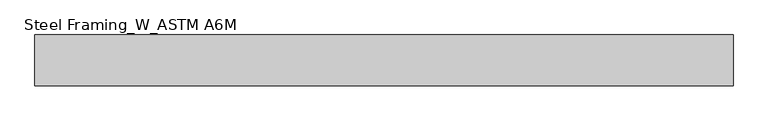
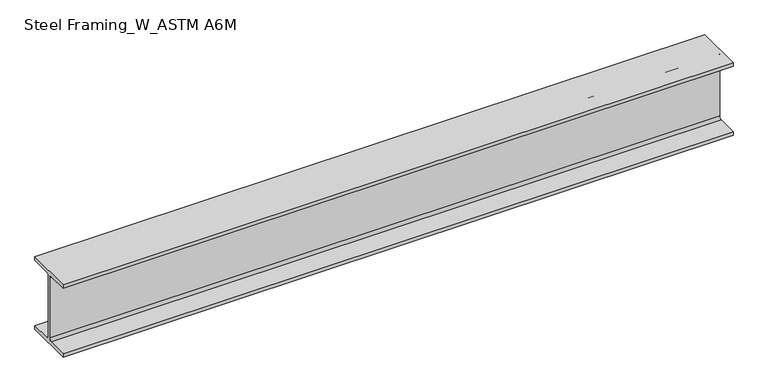
"""IFC4 building model written with IfcOpenShell, lengths in millimetres: beam geometry, Steel Framing_W_ASTM A6M : H_SB_AR_S02_W200x31.3_B6."""

from ifc_helpers import new_model, si_unit, point, frame, frame_2d, origin, place, context, project, spatial, polyline, circle_curve, trimmed, segment, composite_curve, outline, extrude, source, transform, mapped, element, save


def steel_framing_w_astm_a6m_7ac08ae9(model_context):
    return source(origin(), model_context, "Body", "SweptSolid", [
        extrude(outline(composite_curve([segment(polyline([(67.0, -94.8), (67.0, -105.0), (-67.0, -105.0), (-67.0, -94.8), (-10.775, -94.8)]), True, "CONTINUOUS"), segment(trimmed(circle_curve(frame_2d((-10.775, -87.2)), 7.6), [point((-10.775, -94.8))], [point((-3.175, -87.2))], True, "CARTESIAN"), True, "CONTINUOUS"), segment(polyline([(-3.175, -87.2), (-3.175, 87.2)]), True, "CONTINUOUS"), segment(trimmed(circle_curve(frame_2d((-10.775, 87.2)), 7.6), [point((-3.175, 87.2))], [point((-10.775, 94.8))], True, "CARTESIAN"), True, "CONTINUOUS"), segment(polyline([(-10.775, 94.8), (-67.0, 94.8), (-67.0, 105.0), (67.0, 105.0), (67.0, 94.8), (10.775, 94.8)]), True, "CONTINUOUS"), segment(trimmed(circle_curve(frame_2d((10.775, 87.2)), 7.6), [point((10.775, 94.8))], [point((3.175, 87.2))], True, "CARTESIAN"), True, "CONTINUOUS"), segment(polyline([(3.175, 87.2), (3.175, -87.2)]), True, "CONTINUOUS"), segment(trimmed(circle_curve(frame_2d((10.775, -87.2)), 7.6), [point((3.175, -87.2))], [point((10.775, -94.8))], True, "CARTESIAN"), True, "CONTINUOUS"), segment(polyline([(10.775, -94.8), (67.0, -94.8)]), True, "CONTINUOUS")], self_intersect=False)), frame((-920.3, 0.0, 0.0), z_axis=(1.0, 0.0, 0.0), x_axis=(0.0, 1.0, 0.0)), (0.0, 0.0, 1.0), 1840.6),
    ])


if __name__ == "__main__":
    model = new_model("IFC4")
    model_context = context("Model", 3, world=origin())
    ifc_project = project(units=[si_unit("LENGTHUNIT", "METRE", prefix="MILLI")], contexts=[model_context])
    site = spatial("IfcSite", under=ifc_project)
    building = spatial("IfcBuilding", under=site)
    placement = place(None, origin())
    steel_framing_w_astm_a6m_shape = steel_framing_w_astm_a6m_7ac08ae9(model_context)
    element("IfcBeam", 1, ObjectType="Steel Framing_W_ASTM A6M : H_SB_AR_S02_W200x31.3_B6", at=placement, inside=building, context=model_context, shape_type="MappedRepresentation", body=[
        mapped(steel_framing_w_astm_a6m_shape, transform((0.0, 0.0, 0.0), x_axis=(1.0, 0.0, 0.0), y_axis=(0.0, 1.0, 0.0), z_axis=(0.0, 0.0, 1.0))),
    ])
    save(model, "model.ifc")

# Revit data of these elements
# Type "Steel Framing_W_ASTM A6M : H_SB_AR_S02_W200x31.3_B6"
#   Type Mark = "B6"
#   Section Name Key = "W8x21"
#   Width = 13.4 cm
#   Web Thickness = 0.635 cm
#   Web Fillet = 0.76 cm
#   Warping Constant = 40800.0 cm⁶
#   Torsional Moment of Inertia = 11.70 cm⁴
#   Section Area = 39.7 cm²
#   Plastic Modulus weak axis = 93.2 cm³
#   Plastic Modulus strong axis = 334.0 cm³
#   Perimeter = 0.93 m²/m
#   Nominal Weight = 31.30 kgf/m
#   Moment of Inertia weak axis = 407.00 cm⁴
#   Moment of Inertia strong axis = 3130.00 cm⁴
#   Height = 21.0 cm
#   Flange Thickness = 1.02 cm
#   Elastic Modulus weak axis = 60.8 cm³
#   Elastic Modulus strong axis = 298.0 cm³
#   Centroid Vertical = 10.5 cm
#   Centroid Horizontal = 6.7 cm
#   Length [instance default] = 1500 mm
#   Structural Material [instance default] = Steel, 45-345
#   Bolt Spacing = 0
#   Assembly Code = ""
# Element 1 (IfcBeam, "Steel Framing_W_ASTM A6M : H_SB_AR_S02_W200x31.3_B6")
#   Materials on its faces: "Steel, 45-345"
# Materials
#   "Steel, 45-345": class "Metal", colour RGB 189 187 185, transparency 0, Description = "Steel 345 MPa", Cost = 0
